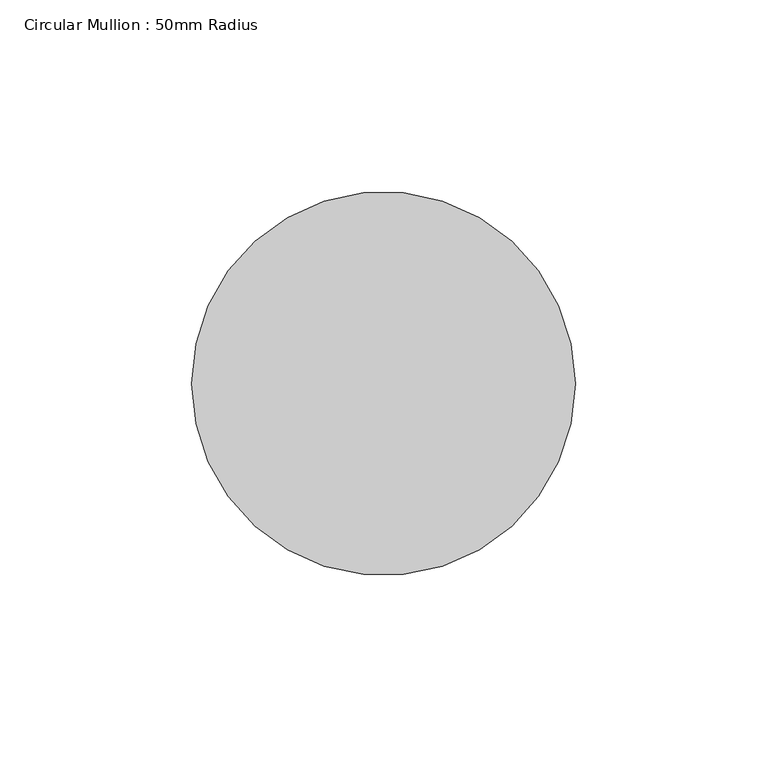
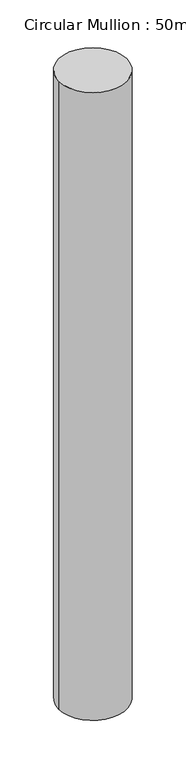
"""IFC4 building model written with IfcOpenShell, lengths in millimetres: member geometry, Circular Mullion : 50mm Radius."""

from ifc_helpers import new_model, si_unit, point, frame, origin, origin_2d, place, context, project, spatial, circle_curve, trimmed, segment, composite_curve, outline, extrude, source, transform, mapped, element, save


def circular_mullion_50mm_radius_e2424c5c(model_context):
    return source(origin(), model_context, "Body", "SweptSolid", [
        extrude(outline(composite_curve([segment(trimmed(circle_curve(origin_2d(), 50.0), [point((50.0, 0.0))], [point((-50.0, 0.0))], False, "CARTESIAN"), True, "CONTINUOUS"), segment(trimmed(circle_curve(origin_2d(), 50.0), [point((-50.0, 0.0))], [point((50.0, 0.0))], False, "CARTESIAN"), True, "CONTINUOUS")], self_intersect=False)), frame((0.0, 0.0, -974.8318761), z_axis=(0.0, 0.0, 1.0), x_axis=(1.0, 0.0, 0.0)), (0.0, 0.0, 1.0), 974.8318761),
    ])


if __name__ == "__main__":
    model = new_model("IFC4")
    model_context = context("Model", 3, world=origin())
    ifc_project = project(units=[si_unit("LENGTHUNIT", "METRE", prefix="MILLI")], contexts=[model_context])
    site = spatial("IfcSite", under=ifc_project)
    building = spatial("IfcBuilding", under=site)
    placement = place(None, origin())
    circular_mullion_50mm_radius_shape = circular_mullion_50mm_radius_e2424c5c(model_context)
    element("IfcMember", 1, ObjectType="Circular Mullion : 50mm Radius", at=placement, inside=building, context=model_context, shape_type="MappedRepresentation", body=[
        mapped(circular_mullion_50mm_radius_shape, transform((0.0, 0.0, 0.0), x_axis=(1.0, 0.0, 0.0), y_axis=(0.0, 1.0, 0.0), z_axis=(0.0, 0.0, 1.0))),
    ])
    save(model, "model.ifc")

# Revit data of these elements
# Type "Circular Mullion : 50mm Radius"
#   built-in parameter 1007350 = 0.164042 (stored number, unit not read)
# Element 1 (IfcMember, "Circular Mullion : 50mm Radius")
#   Materials on its faces: "Aluminium"
# Materials
#   "Aluminium": class "Metal", colour RGB 247 247 247, transparency 0, Description = "Aluminium 6061", Cost = 0
